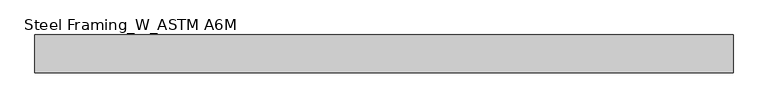
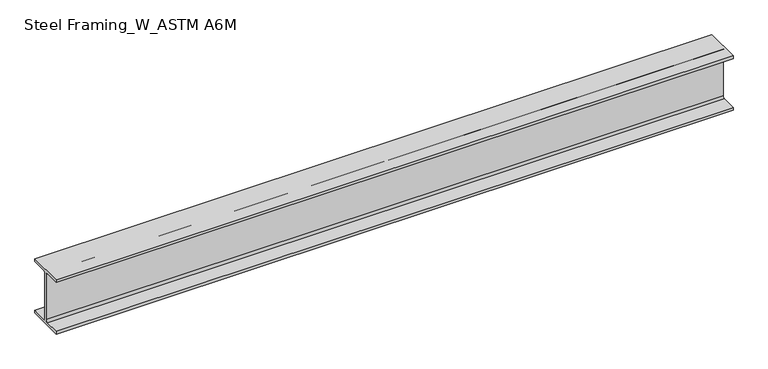
"""IFC4 building model written with IfcOpenShell, lengths in millimetres: beam geometry, Steel Framing_W_ASTM A6M : H_SB_AR_S02_W200x31.3_B6."""

from ifc_helpers import new_model, si_unit, point, frame, frame_2d, origin, place, context, project, spatial, polyline, circle_curve, trimmed, segment, composite_curve, outline, extrude, source, transform, mapped, element, save


def steel_framing_w_astm_a6m_85c0693e(model_context):
    return source(origin(), model_context, "Body", "SweptSolid", [
        extrude(outline(composite_curve([segment(polyline([(67.0, -94.8), (67.0, -105.0), (-67.0, -105.0), (-67.0, -94.8), (-10.775, -94.8)]), True, "CONTINUOUS"), segment(trimmed(circle_curve(frame_2d((-10.775, -87.2)), 7.6), [point((-10.775, -94.8))], [point((-3.175, -87.2))], True, "CARTESIAN"), True, "CONTINUOUS"), segment(polyline([(-3.175, -87.2), (-3.175, 87.2)]), True, "CONTINUOUS"), segment(trimmed(circle_curve(frame_2d((-10.775, 87.2)), 7.6), [point((-3.175, 87.2))], [point((-10.775, 94.8))], True, "CARTESIAN"), True, "CONTINUOUS"), segment(polyline([(-10.775, 94.8), (-67.0, 94.8), (-67.0, 105.0), (67.0, 105.0), (67.0, 94.8), (10.775, 94.8)]), True, "CONTINUOUS"), segment(trimmed(circle_curve(frame_2d((10.775, 87.2)), 7.6), [point((10.775, 94.8))], [point((3.175, 87.2))], True, "CARTESIAN"), True, "CONTINUOUS"), segment(polyline([(3.175, 87.2), (3.175, -87.2)]), True, "CONTINUOUS"), segment(trimmed(circle_curve(frame_2d((10.775, -87.2)), 7.6), [point((3.175, -87.2))], [point((10.775, -94.8))], True, "CARTESIAN"), True, "CONTINUOUS"), segment(polyline([(10.775, -94.8), (67.0, -94.8)]), True, "CONTINUOUS")], self_intersect=False)), frame((-1236.4, 0.0, 0.0), z_axis=(1.0, 0.0, 0.0), x_axis=(0.0, 1.0, 0.0)), (0.0, 0.0, 1.0), 2472.8),
    ])


if __name__ == "__main__":
    model = new_model("IFC4")
    model_context = context("Model", 3, world=origin())
    ifc_project = project(units=[si_unit("LENGTHUNIT", "METRE", prefix="MILLI")], contexts=[model_context])
    site = spatial("IfcSite", under=ifc_project)
    building = spatial("IfcBuilding", under=site)
    placement = place(None, origin())
    steel_framing_w_astm_a6m_shape = steel_framing_w_astm_a6m_85c0693e(model_context)
    element("IfcBeam", 1, ObjectType="Steel Framing_W_ASTM A6M : H_SB_AR_S02_W200x31.3_B6", at=placement, inside=building, context=model_context, shape_type="MappedRepresentation", body=[
        mapped(steel_framing_w_astm_a6m_shape, transform((0.0, 0.0, 0.0), x_axis=(1.0, 0.0, 0.0), y_axis=(0.0, 1.0, 0.0), z_axis=(0.0, 0.0, 1.0))),
    ])
    save(model, "model.ifc")

# Revit data of these elements
# Type "Steel Framing_W_ASTM A6M : H_SB_AR_S02_W200x31.3_B6"
#   Type Mark = "B6"
#   Section Name Key = "W8x21"
#   Width = 13.4 cm
#   Web Thickness = 0.635 cm
#   Web Fillet = 0.76 cm
#   Warping Constant = 40800.0 cm⁶
#   Torsional Moment of Inertia = 11.70 cm⁴
#   Section Area = 39.7 cm²
#   Plastic Modulus weak axis = 93.2 cm³
#   Plastic Modulus strong axis = 334.0 cm³
#   Perimeter = 0.93 m²/m
#   Nominal Weight = 31.30 kgf/m
#   Moment of Inertia weak axis = 407.00 cm⁴
#   Moment of Inertia strong axis = 3130.00 cm⁴
#   Height = 21.0 cm
#   Flange Thickness = 1.02 cm
#   Elastic Modulus weak axis = 60.8 cm³
#   Elastic Modulus strong axis = 298.0 cm³
#   Centroid Vertical = 10.5 cm
#   Centroid Horizontal = 6.7 cm
#   Length [instance default] = 1500 mm
#   Structural Material [instance default] = Steel, 45-345
#   Bolt Spacing = 0
#   Assembly Code = ""
# Element 1 (IfcBeam, "Steel Framing_W_ASTM A6M : H_SB_AR_S02_W200x31.3_B6")
#   Materials on its faces: "Steel, 45-345"
# Materials
#   "Steel, 45-345": class "Metal", colour RGB 189 187 185, transparency 0, Description = "Steel 345 MPa", Cost = 0
